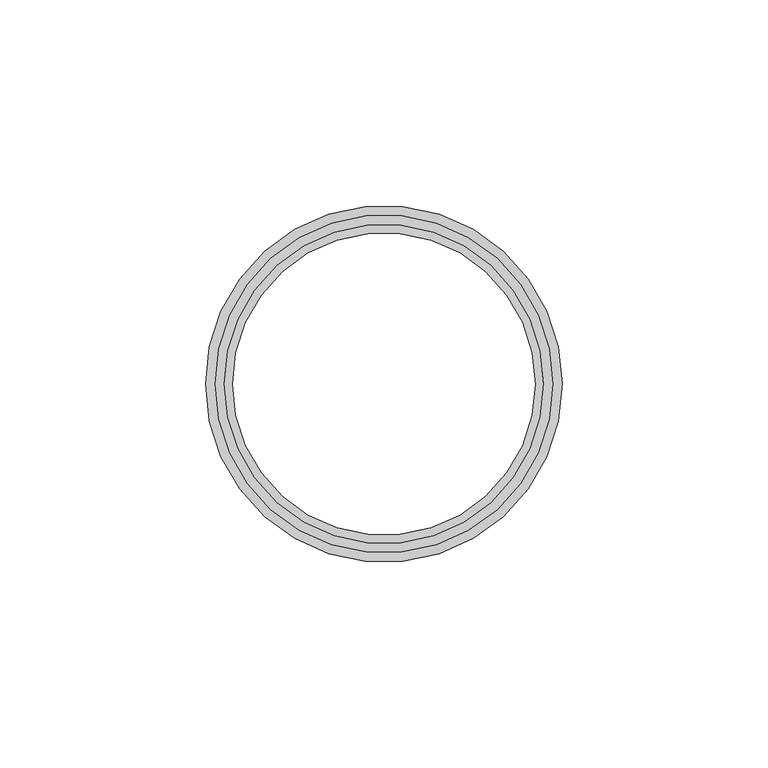
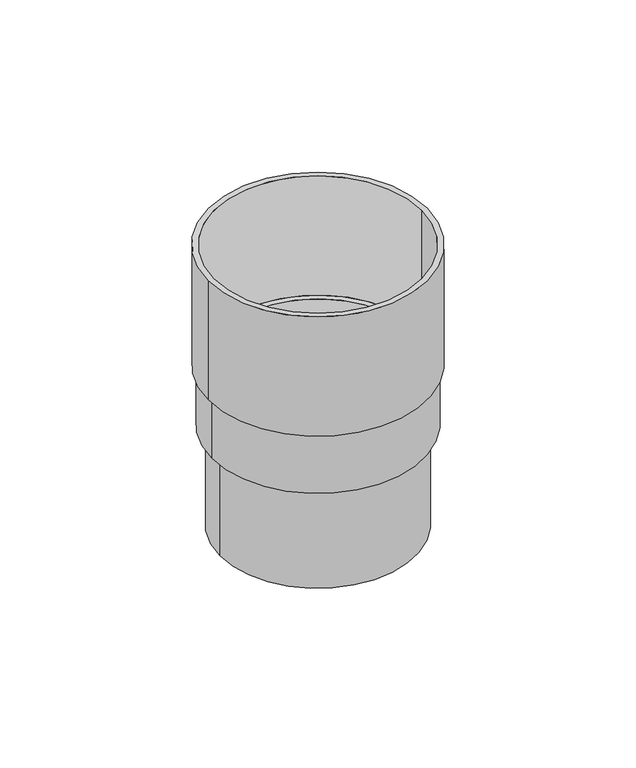
"""IFC4 building model written with IfcOpenShell, lengths in millimetres: proxy geometry, ⇱ Соеденительная муфта с хомутом крепления трубы : ⇱ Соеденительная муфта с хомутом крепления трубы."""

from ifc_helpers import new_model, si_unit, frame, origin, origin_with_axes, place, context, project, spatial, polyline, circle_curve, source, transform, mapped, element, save
from ifc_brep_helpers import plane_surface, cylinder_surface, revolved_surface, advanced_brep


def generic_models_4bd52057(model_context):
    return source(origin(), model_context, "Body", "AdvancedBrep", [
        advanced_brep(
        [(-43.4, 0.0, 0.0), (43.4, 0.0, 0.0), (-41.1, 0.0, 0.0), (41.1, 0.0, 0.0), (-43.4, 0.0, -50.0), (43.4, 0.0, -50.0), (-42.0, 0.0, -50.0), (42.0, 0.0, -50.0), (-41.1, 0.0, -50.0), (41.1, 0.0, -50.0), (-38.8, 0.0, -50.0), (38.8, 0.0, -50.0), (-42.0, 0.0, -75.0), (42.0, 0.0, -75.0), (-38.8, 0.0, -75.0), (38.8, 0.0, -75.0), (-38.8, 0.0, -75.0), (38.8, 0.0, -75.0), (-36.8, 0.0, -75.0), (36.8, 0.0, -75.0), (-38.8, 0.0, -117.0), (38.8, 0.0, -117.0), (-36.8, 0.0, -117.0), (36.8, 0.0, -117.0)],
        [
            (0, 1, circle_curve(origin_with_axes(), 43.4)),
            (1, 0, circle_curve(origin_with_axes(), 43.4)),
            (2, 3, circle_curve(frame((0.0, 0.0, 0.0), z_axis=(0.0, 0.0, -1.0), x_axis=(1.0, 0.0, 0.0)), 41.1)),
            (3, 2, circle_curve(frame((0.0, 0.0, 0.0), z_axis=(0.0, 0.0, -1.0), x_axis=(1.0, 0.0, 0.0)), 41.1)),
            (4, 5, circle_curve(frame((0.0, 0.0, -50.0), z_axis=(0.0, 0.0, -1.0), x_axis=(1.0, 0.0, 0.0)), 43.4)),
            (5, 4, circle_curve(frame((0.0, 0.0, -50.0), z_axis=(0.0, 0.0, -1.0), x_axis=(1.0, 0.0, 0.0)), 43.4)),
            (6, 7, circle_curve(frame((0.0, 0.0, -50.0), z_axis=(0.0, 0.0, 1.0), x_axis=(1.0, 0.0, 0.0)), 42.0)),
            (7, 6, circle_curve(frame((0.0, 0.0, -50.0), z_axis=(0.0, 0.0, 1.0), x_axis=(1.0, 0.0, 0.0)), 42.0)),
            (2, 8),
            (8, 9, circle_curve(frame((0.0, 0.0, -50.0), z_axis=(0.0, 0.0, -1.0), x_axis=(1.0, 0.0, 0.0)), 41.1)),
            (9, 3),
            (9, 8, circle_curve(frame((0.0, 0.0, -50.0), z_axis=(0.0, 0.0, -1.0), x_axis=(1.0, 0.0, 0.0)), 41.1)),
            (0, 4),
            (5, 1),
            (10, 11, circle_curve(frame((0.0, 0.0, -50.0), z_axis=(0.0, 0.0, -1.0), x_axis=(1.0, 0.0, 0.0)), 38.8)),
            (11, 10, circle_curve(frame((0.0, 0.0, -50.0), z_axis=(0.0, 0.0, -1.0), x_axis=(1.0, 0.0, 0.0)), 38.8)),
            (12, 13, circle_curve(frame((0.0, 0.0, -75.0), z_axis=(0.0, 0.0, -1.0), x_axis=(1.0, 0.0, 0.0)), 42.0)),
            (13, 12, circle_curve(frame((0.0, 0.0, -75.0), z_axis=(0.0, 0.0, -1.0), x_axis=(1.0, 0.0, 0.0)), 42.0)),
            (14, 15, circle_curve(frame((0.0, 0.0, -75.0), z_axis=(0.0, 0.0, 1.0), x_axis=(1.0, 0.0, 0.0)), 38.8)),
            (15, 14, circle_curve(frame((0.0, 0.0, -75.0), z_axis=(0.0, 0.0, 1.0), x_axis=(1.0, 0.0, 0.0)), 38.8)),
            (10, 16),
            (16, 17, circle_curve(frame((0.0, 0.0, -75.0), z_axis=(0.0, 0.0, -1.0), x_axis=(1.0, 0.0, 0.0)), 38.8)),
            (17, 11),
            (17, 16, circle_curve(frame((0.0, 0.0, -75.0), z_axis=(0.0, 0.0, -1.0), x_axis=(1.0, 0.0, 0.0)), 38.8)),
            (13, 7),
            (6, 12),
            (18, 19, circle_curve(frame((0.0, 0.0, -75.0), z_axis=(0.0, 0.0, -1.0), x_axis=(1.0, 0.0, 0.0)), 36.8)),
            (19, 18, circle_curve(frame((0.0, 0.0, -75.0), z_axis=(0.0, 0.0, -1.0), x_axis=(1.0, 0.0, 0.0)), 36.8)),
            (20, 21, circle_curve(frame((0.0, 0.0, -117.0), z_axis=(0.0, 0.0, -1.0), x_axis=(1.0, 0.0, 0.0)), 38.8)),
            (21, 20, circle_curve(frame((0.0, 0.0, -117.0), z_axis=(0.0, 0.0, -1.0), x_axis=(1.0, 0.0, 0.0)), 38.8)),
            (22, 23, circle_curve(frame((0.0, 0.0, -117.0), z_axis=(0.0, 0.0, 1.0), x_axis=(1.0, 0.0, 0.0)), 36.8)),
            (23, 22, circle_curve(frame((0.0, 0.0, -117.0), z_axis=(0.0, 0.0, 1.0), x_axis=(1.0, 0.0, 0.0)), 36.8)),
            (18, 22),
            (23, 19),
            (21, 15),
            (14, 20),
        ],
        [
            plane_surface(frame((41.1, 0.0, 0.0), z_axis=(0.0, 0.0, 1.0), x_axis=(0.0, -1.0, 0.0))),
            plane_surface(frame((41.1, 0.0, -50.0), z_axis=(0.0, 0.0, -1.0), x_axis=(0.0, 1.0, 0.0))),
            revolved_surface(polyline([(41.1, 0.0, -50.0), (41.1, 0.0, 0.0)]), (0.0, 0.0, -50.0), (0.0, 0.0, -1.0)),
            cylinder_surface(origin_with_axes(), 43.4),
            plane_surface(frame((38.8, 0.0, -50.0), z_axis=(0.0, 0.0, 1.0), x_axis=(0.0, -1.0, 0.0))),
            plane_surface(frame((38.8, 0.0, -75.0), z_axis=(0.0, 0.0, -1.0), x_axis=(0.0, 1.0, 0.0))),
            revolved_surface(polyline([(38.8, 0.0, -75.0), (38.8, 0.0, -50.0)]), (0.0, 0.0, -75.0), (0.0, 0.0, -1.0)),
            cylinder_surface(origin_with_axes(), 42.0),
            plane_surface(frame((36.8, 0.0, -75.0), z_axis=(0.0, 0.0, 1.0), x_axis=(0.0, -1.0, 0.0))),
            plane_surface(frame((36.8, 0.0, -117.0), z_axis=(0.0, 0.0, -1.0), x_axis=(0.0, 1.0, 0.0))),
            revolved_surface(polyline([(36.8, 0.0, -117.0), (36.8, 0.0, -75.0)]), (0.0, 0.0, -117.0), (0.0, 0.0, -1.0)),
            cylinder_surface(frame((0.0, 0.0, -32.655027), z_axis=(0.0, 0.0, 1.0), x_axis=(1.0, 0.0, 0.0)), 38.8),
        ],
        [
            (0, [[1, 2], [3, 4]]),
            (1, [[5, 6], [7, 8]]),
            (2, [[-3, 9, 10, 11]]),
            (2, [[-4, -11, 12, -9]]),
            (3, [[-1, 13, -6, 14]]),
            (3, [[-2, -14, -5, -13]]),
            (4, [[-10, -12], [15, 16]]),
            (5, [[17, 18], [19, 20]]),
            (6, [[-15, 21, 22, 23]]),
            (6, [[-16, -23, 24, -21]]),
            (7, [[-18, 25, -7, 26]]),
            (7, [[-17, -26, -8, -25]]),
            (8, [[-22, -24], [27, 28]]),
            (9, [[29, 30], [31, 32]]),
            (10, [[-27, 33, -32, 34]]),
            (10, [[-28, -34, -31, -33]]),
            (11, [[-30, 35, -19, 36]]),
            (11, [[-29, -36, -20, -35]]),
        ],
    ),
    ])


if __name__ == "__main__":
    model = new_model("IFC4")
    model_context = context("Model", 3, world=origin())
    ifc_project = project(units=[si_unit("LENGTHUNIT", "METRE", prefix="MILLI")], contexts=[model_context])
    site = spatial("IfcSite", under=ifc_project)
    building = spatial("IfcBuilding", under=site)
    placement = place(None, origin())
    generic_models_shape = generic_models_4bd52057(model_context)
    element("IfcBuildingElementProxy", 1, Name="⇱ Соеденительная муфта с хомутом крепления трубы : ⇱ Соеденительная муфта с хомутом крепления трубы", ObjectType="⇱ Соеденительная муфта с хомутом крепления трубы : ⇱ Соеденительная муфта с хомутом крепления трубы", at=placement, inside=building, context=model_context, shape_type="MappedRepresentation", body=[
        mapped(generic_models_shape, transform((0.0, 0.0, 0.0), x_axis=(1.0, 0.0, 0.0), y_axis=(0.0, 1.0, 0.0), z_axis=(0.0, 0.0, 1.0))),
    ])
    save(model, "model.ifc")

# Revit data of these elements
# Type "⇱ Соеденительная муфта с хомутом крепления трубы : ⇱ Соеденительная муфта с хомутом крепления трубы"
#   Description = "Обеспечивает соединение водосточных\r\nтруб, компенсирует температурное расширение"
#   Manufacturer = "ТехноНИКОЛЬ"
#   Model = "Комплектующие к водосточным системам"
#   URL = "https://tn-vodostok.ru/catalog/pvh/"
#   ADSK_Обозначение = "ТехноНИКОЛЬ"
#   ADSK_Наименование краткое = "Муфта"
#   ADSK_Наименование = "Соединительная муфта"
#   ADSK_Масса_Текст = ""
#   ADSK_Марка = ""
#   ADSK_Код изделия = ""
#   ADSK_Завод-изготовитель = "ТехноНИКОЛЬ"
#   ADSK_Единица измерения = "шт."
#   ADSK_Группирование = "Комплектующие к водосточным системам"
#   ADSK_URL страницы изделия = "https://tn-vodostok.ru/catalog/pvh/"
#   ADSK_URL документации изделия = "https://tn-vodostok.ru/upload/iblock/c42/c427963cb77eb5c3c51f0cfb870e9e52.pdf"
#   ADSK_Размер_Ширина = 86.8 mm
#   ADSK_Размер_Диаметр = 82.2 mm
#   ADSK_Размер_Высота = 117 mm
#   ADSK_Количество = 1
#   ADSK_Материал [instance default] = TN_Пластик_Коричневый_RAL8019
#   Default Elevation = 0
# Element 1 (IfcBuildingElementProxy, "⇱ Соеденительная муфта с хомутом крепления трубы : ⇱ Соеденительная муфта с хомутом крепления трубы")
#   Materials on its faces: "TN_Пластик_Коричневый_RAL8019"
# Materials
#   "TN_Пластик_Коричневый_RAL8019": class "Типовые", colour RGB 61 54 53, transparency 0, Cost = 0
